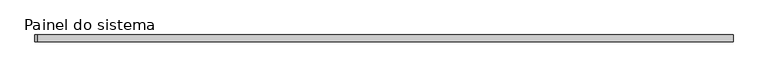
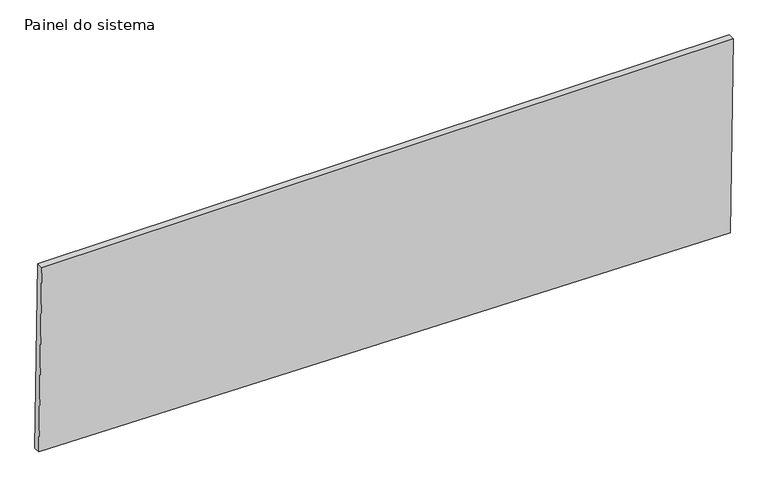
"""IFC4 building model written with IfcOpenShell, lengths in millimetres: plate geometry, Painel do sistema : Envidraçado."""

from ifc_helpers import new_model, si_unit, frame, origin, place, context, project, spatial, polyline, outline, extrude, source, transform, mapped, element, save


def painel_do_sistema_78fe6786(model_context):
    return source(origin(), model_context, "Body", "SweptSolid", [
        extrude(outline(polyline([(37.9368749, -1266.7735904), (0.0, 1255.5700723), (744.8985412, 1266.7735904), (744.8985412, -1256.1406554), (37.9368749, -1266.7735904)])), frame((0.0, 24.5, 0.0), z_axis=(0.0, 1.0, 0.0), x_axis=(0.0, 0.0, 1.0)), (0.0, 0.0, 1.0), 25.0),
    ])


if __name__ == "__main__":
    model = new_model("IFC4")
    model_context = context("Model", 3, world=origin())
    ifc_project = project(units=[si_unit("LENGTHUNIT", "METRE", prefix="MILLI")], contexts=[model_context])
    site = spatial("IfcSite", under=ifc_project)
    building = spatial("IfcBuilding", under=site)
    placement = place(None, origin())
    painel_do_sistema_shape = painel_do_sistema_78fe6786(model_context)
    element("IfcPlate", 1, ObjectType="Painel do sistema : Envidraçado", at=placement, inside=building, context=model_context, shape_type="MappedRepresentation", body=[
        mapped(painel_do_sistema_shape, transform((0.0, 0.0, 0.0), x_axis=(1.0, 0.0, 0.0), y_axis=(0.0, 1.0, 0.0), z_axis=(0.0, 0.0, 1.0))),
    ])
    save(model, "model.ifc")

# Revit data of these elements
# Type "Painel do sistema : Envidraçado"
#   Construction Type Id = "GSP4R"
#   Analytic Construction = "Vidraça única Pilkington 1/8 pol"
#   Visual Light Transmittance = 0.9
#   Solar Heat Gain Coefficient = 0.86
#   Heat Transfer Coefficient (U) = 6.7069 W/(m²·K)
# Element 1 (IfcPlate, "Painel do sistema : Envidraçado")
#   Materials on its faces: "Vidro"
# Materials
#   "Vidro": class "Vidro", colour RGB 0 128 192, transparency 0.9, Description = "Vidro de sílica", Cost = 0
